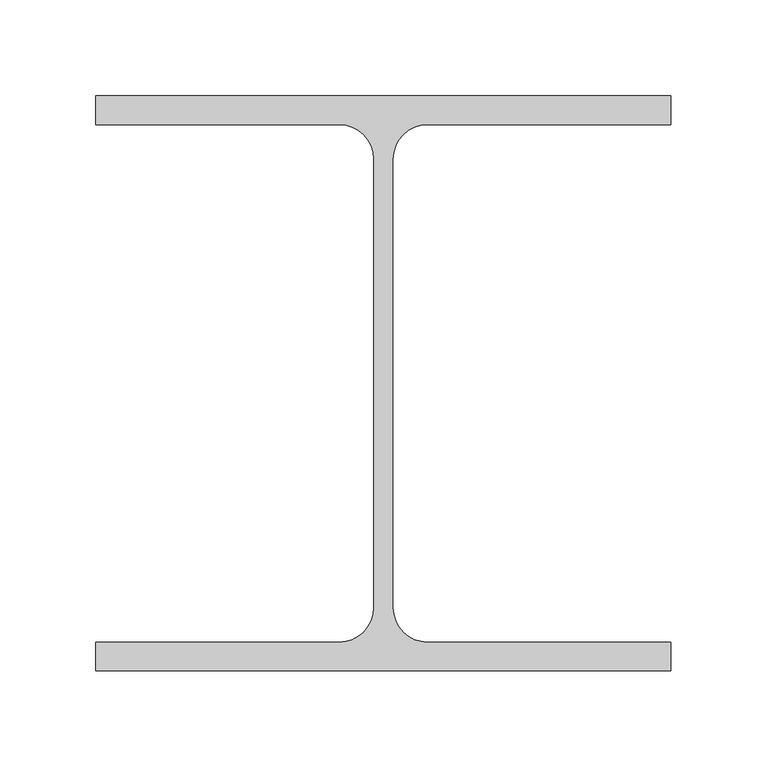
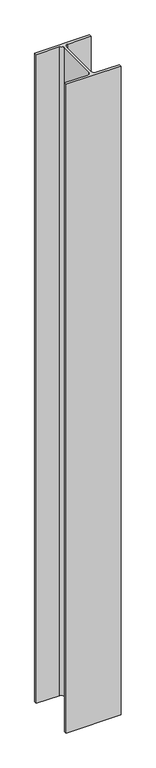
"""IFC4 building model written with IfcOpenShell, lengths in millimetres: column geometry, 0912_Steel Column_H_KSD3502 : H_SC_ASC_H-300x300x10x15."""

from ifc_helpers import new_model, si_unit, point, frame, frame_2d, origin, place, context, project, spatial, polyline, circle_curve, trimmed, segment, composite_curve, outline, extrude, source, transform, mapped, element, save


def column_2bf4f364(model_context):
    return source(origin(), model_context, "Body", "SweptSolid", [
        extrude(outline(composite_curve([segment(polyline([(150.0, 150.0), (150.0, 135.0), (23.0, 135.0)]), True, "CONTINUOUS"), segment(trimmed(circle_curve(frame_2d((23.0, 117.0)), 18.0), [point((23.0, 135.0))], [point((5.0, 117.0))], True, "CARTESIAN"), True, "CONTINUOUS"), segment(polyline([(5.0, 117.0), (5.0, -117.0)]), True, "CONTINUOUS"), segment(trimmed(circle_curve(frame_2d((23.0, -117.0)), 18.0), [point((5.0, -117.0))], [point((23.0, -135.0))], True, "CARTESIAN"), True, "CONTINUOUS"), segment(polyline([(23.0, -135.0), (150.0, -135.0), (150.0, -150.0), (-150.0, -150.0), (-150.0, -135.0), (-23.0, -135.0)]), True, "CONTINUOUS"), segment(trimmed(circle_curve(frame_2d((-23.0, -117.0)), 18.0), [point((-23.0, -135.0))], [point((-5.0, -117.0))], True, "CARTESIAN"), True, "CONTINUOUS"), segment(polyline([(-5.0, -117.0), (-5.0, 117.0)]), True, "CONTINUOUS"), segment(trimmed(circle_curve(frame_2d((-23.0, 117.0)), 18.0), [point((-5.0, 117.0))], [point((-23.0, 135.0))], True, "CARTESIAN"), True, "CONTINUOUS"), segment(polyline([(-23.0, 135.0), (-150.0, 135.0), (-150.0, 150.0), (150.0, 150.0)]), True, "CONTINUOUS")], self_intersect=False)), frame((0.0, 0.0, 685.9720055), z_axis=(0.0, 0.0, 1.0), x_axis=(1.0, 0.0, 0.0)), (0.0, 0.0, 1.0), 3764.0),
    ])


if __name__ == "__main__":
    model = new_model("IFC4")
    model_context = context("Model", 3, world=origin())
    ifc_project = project(units=[si_unit("LENGTHUNIT", "METRE", prefix="MILLI")], contexts=[model_context])
    site = spatial("IfcSite", under=ifc_project)
    building = spatial("IfcBuilding", under=site)
    placement = place(None, origin())
    column_shape = column_2bf4f364(model_context)
    element("IfcColumn", 1, ObjectType="0912_Steel Column_H_KSD3502 : H_SC_ASC_H-300x300x10x15", at=placement, inside=building, context=model_context, shape_type="MappedRepresentation", body=[
        mapped(column_shape, transform((0.0, 0.0, 0.0), x_axis=(1.0, 0.0, 0.0), y_axis=(0.0, 1.0, 0.0), z_axis=(0.0, 0.0, 1.0))),
    ])
    save(model, "model.ifc")

# Revit data of these elements
# Type "0912_Steel Column_H_KSD3502 : H_SC_ASC_H-300x300x10x15"
#   H_WM Code_1 = "S01AA002-00001 | Main Steel Structure Fabrication Work | Shelter/Building | Medium Steel - Standard (90KG/M>Weight≥30KG/M) | Material: (   )"
#   H_WM Code_2 = "S03AA028-00001 | Main Steel Structure Erection Work | Shelter/Building | Medium Steel (90KG/M>Weight≥30KG/M) | Material: (   )"
#   H_WM Code_3 = "S01AA010-00001 | Main Steel Structure Fabrication Work | Shelter/Building | Steel Painting/Coating | for Non-Fireproofed Steel Surface, Surface Preparation, Primer, Second & Final Coat | Material: (   )"
#   H_Q'ty Cal Type Tag = "SC-Q2"
#   Width = 30.0 cm
#   Web Thickness = 1.0 cm
#   Web Fillet = 1.8 cm
#   Warping Constant = 1370670.0 cm⁶
#   Torsional Moment of Inertia = 77.00 cm⁴
#   Section Area = 119.8 cm²
#   Plastic Modulus weak axis = 684.0 cm³
#   Plastic Modulus strong axis = 1500.0 cm³
#   Perimeter = 1.75 m²/m
#   Nominal Weight = 94.00 kgf/m
#   Moment of Inertia weak axis = 6750.00 cm⁴
#   Moment of Inertia strong axis = 20400.00 cm⁴
#   Height = 30.0 cm
#   Flange Thickness = 1.5 cm
#   Elastic Modulus weak axis = 450.0 cm³
#   Elastic Modulus strong axis = 1360.0 cm³
#   Centroid Vertical = 15.0 cm
#   Centroid Horizontal = 15.0 cm
#   Structural Material [instance default] = Steel, 45-345
#   Section Name Key = ""
#   Bolt Spacing = 0
#   Assembly Code = ""
# Element 1 (IfcColumn, "0912_Steel Column_H_KSD3502 : H_SC_ASC_H-300x300x10x15")
#   Structural Material = none
# Materials
#   "Steel, 45-345": class "Metal", colour RGB 189 187 185, transparency 0, Description = "Steel 345 MPa", Cost = 0
